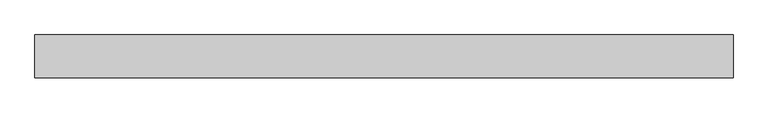
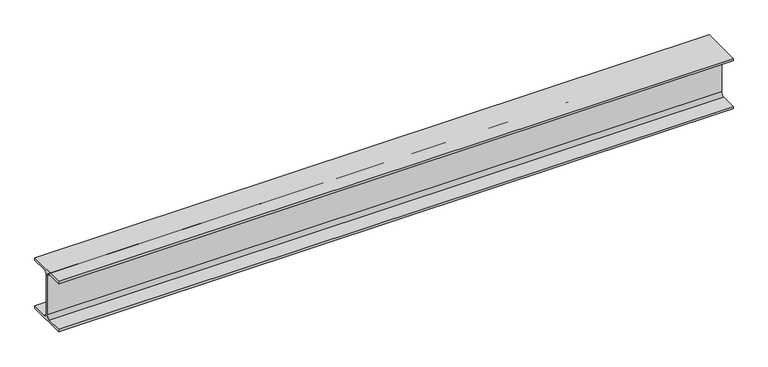
"""IFC4 building model written with IfcOpenShell, lengths in millimetres: beam geometry, 0912_Steel Framing_H-KSD3502 : H_SB_ASB_H-194x150x6x9."""

from ifc_helpers import new_model, si_unit, point, frame, frame_2d, origin, place, context, project, spatial, polyline, circle_curve, trimmed, segment, composite_curve, outline, extrude, source, transform, mapped, element, save


def beam_fea0a2c5(model_context):
    return source(origin(), model_context, "Body", "SweptSolid", [
        extrude(outline(composite_curve([segment(polyline([(-75.0, -88.0), (-16.0, -88.0)]), True, "CONTINUOUS"), segment(trimmed(circle_curve(frame_2d((-16.0, -75.0)), 13.0), [point((-16.0, -88.0))], [point((-3.0, -75.0))], True, "CARTESIAN"), True, "CONTINUOUS"), segment(polyline([(-3.0, -75.0), (-3.0, 75.0)]), True, "CONTINUOUS"), segment(trimmed(circle_curve(frame_2d((-16.0, 75.0)), 13.0), [point((-3.0, 75.0))], [point((-16.0, 88.0))], True, "CARTESIAN"), True, "CONTINUOUS"), segment(polyline([(-16.0, 88.0), (-75.0, 88.0), (-75.0, 97.0), (75.0, 97.0), (75.0, 88.0), (16.0, 88.0)]), True, "CONTINUOUS"), segment(trimmed(circle_curve(frame_2d((16.0, 75.0)), 13.0), [point((16.0, 88.0))], [point((3.0, 75.0))], True, "CARTESIAN"), True, "CONTINUOUS"), segment(polyline([(3.0, 75.0), (3.0, -75.0)]), True, "CONTINUOUS"), segment(trimmed(circle_curve(frame_2d((16.0, -75.0)), 13.0), [point((3.0, -75.0))], [point((16.0, -88.0))], True, "CARTESIAN"), True, "CONTINUOUS"), segment(polyline([(16.0, -88.0), (75.0, -88.0), (75.0, -97.0), (-75.0, -97.0), (-75.0, -88.0)]), True, "CONTINUOUS")], self_intersect=False)), frame((-1200.0, 0.0, 0.0), z_axis=(1.0, 0.0, 0.0), x_axis=(0.0, 1.0, 0.0)), (0.0, 0.0, 1.0), 2453.7727018),
    ])


if __name__ == "__main__":
    model = new_model("IFC4")
    model_context = context("Model", 3, world=origin())
    ifc_project = project(units=[si_unit("LENGTHUNIT", "METRE", prefix="MILLI")], contexts=[model_context])
    site = spatial("IfcSite", under=ifc_project)
    building = spatial("IfcBuilding", under=site)
    placement = place(None, origin())
    beam_shape = beam_fea0a2c5(model_context)
    element("IfcBeam", 1, ObjectType="0912_Steel Framing_H-KSD3502 : H_SB_ASB_H-194x150x6x9", at=placement, inside=building, context=model_context, shape_type="MappedRepresentation", body=[
        mapped(beam_shape, transform((0.0, 0.0, 0.0), x_axis=(1.0, 0.0, 0.0), y_axis=(0.0, 1.0, 0.0), z_axis=(0.0, 0.0, 1.0))),
    ])
    save(model, "model.ifc")

# Revit data of these elements
# Type "0912_Steel Framing_H-KSD3502 : H_SB_ASB_H-194x150x6x9"
#   H_WM Code_1 = "S01AA002-00001 | Main Steel Structure Fabrication Work | Shelter/Building | Medium Steel - Standard (90KG/M>Weight≥30KG/M) | Material: (   )"
#   H_WM Code_2 = "S03AA028-00001 | Main Steel Structure Erection Work | Shelter/Building | Medium Steel (90KG/M>Weight≥30KG/M) | Material: (   )"
#   H_WM Code_3 = "S01AA010-00001 | Main Steel Structure Fabrication Work | Shelter/Building | Steel Painting/Coating | for Non-Fireproofed Steel Surface, Surface Preparation, Primer, Second & Final Coat | Material: (   )"
#   H_Q'ty Cal Type Tag = "SB-Q2"
#   Width = 15.0 cm
#   Web Thickness = 0.6 cm
#   Web Fillet = 1.3 cm
#   Warping Constant = 43316.0 cm⁶
#   W = 0
#   Torsional Moment of Inertia = 8.622 cm⁴
#   Section Area = 39.01 cm²
#   Plastic Modulus weak axis = 104.0 cm³
#   Plastic Modulus strong axis = 309.0 cm³
#   Perimeter = 0.95 m²/m
#   Nominal Weight = 30.60 kgf/m
#   Moment of Inertia weak axis = 507.00 cm⁴
#   Moment of Inertia strong axis = 2690.00 cm⁴
#   Height = 19.4 cm
#   Flange Thickness = 0.9 cm
#   Elastic Modulus weak axis = 67.6 cm³
#   Elastic Modulus strong axis = 277.0 cm³
#   Centroid Vertical = 9.7 cm
#   Centroid Horizontal = 7.5 cm
#   Ix = 26900000
#   Length [instance default] = 1.5240 m
#   Zx = 309000
#   b = 0.1500 m
#   h = 0.1940 m
#   r = 0.0130 m
#   s = 0.0060 m
#   t = 0.0090 m
#   A = 0.003901 m²
#   Structural Material [instance default] = Steel, 45-345
#   Assembly Code = ""
# Element 1 (IfcBeam, "0912_Steel Framing_H-KSD3502 : H_SB_ASB_H-194x150x6x9")
#   Structural Material = none
# Materials
#   "Steel, 45-345": class "Metal", colour RGB 189 187 185, transparency 0, Description = "Steel 345 MPa", Cost = 0
